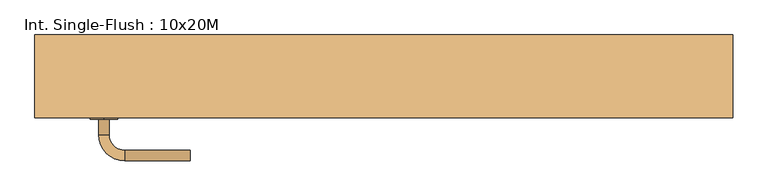
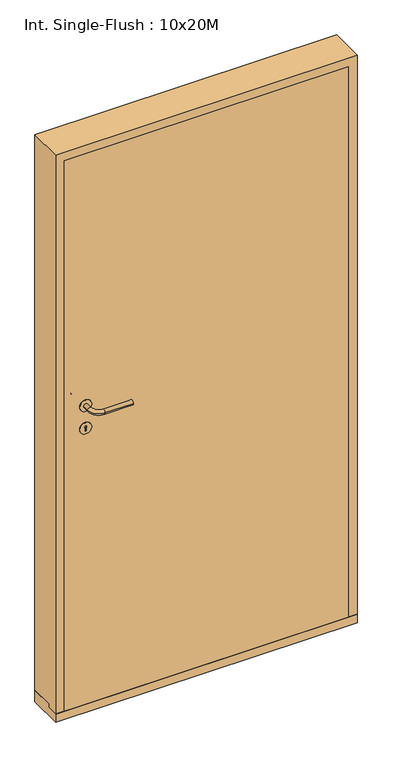
"""IFC4 building model written with IfcOpenShell, lengths in millimetres: door geometry, Int. Single-Flush : 10x20M."""

from ifc_helpers import new_model, si_unit, point, frame, frame_2d, origin, place, context, project, spatial, polyline, circle_curve, ellipse_curve, trimmed, segment, composite_curve, outline, extrude, faceted_brep, source, transform, mapped, element, save
from ifc_brep_helpers import plane_surface, cylinder_surface, revolved_surface, advanced_brep


def int_single_flush_10x20m_68751a9d(model_context):
    return source(origin(), model_context, "Body", "SolidModel", [
        extrude(outline(composite_curve([segment(trimmed(circle_curve(frame_2d((1090.0, -406.0)), 20.0), [point((1070.0, -406.0))], [point((1110.0, -406.0))], False, "CARTESIAN"), True, "CONTINUOUS"), segment(trimmed(circle_curve(frame_2d((1090.0, -406.0)), 20.0), [point((1110.0, -406.0))], [point((1070.0, -406.0))], False, "CARTESIAN"), True, "CONTINUOUS")], self_intersect=False)), frame((0.0, -62.0, 0.0), z_axis=(0.0, 1.0, 0.0), x_axis=(0.0, 0.0, 1.0)), (0.0, 0.0, 1.0), 2.0),
        advanced_brep(
        [(-413.5, -62.0, 1090.0), (-398.5, -62.0, 1090.0), (-398.5, -84.5, 1090.0), (-413.5, -84.5, 1090.0), (-376.0, -107.0, 1090.0), (-376.0, -122.0, 1090.0), (-281.0, -107.0, 1090.0), (-281.0, -122.0, 1090.0)],
        [
            (0, 1, circle_curve(frame((-406.0, -62.0, 1090.0), z_axis=(0.0, 1.0, 0.0), x_axis=(1.0, 0.0, 0.0)), 7.5)),
            (1, 0, circle_curve(frame((-406.0, -62.0, 1090.0), z_axis=(0.0, 1.0, 0.0), x_axis=(1.0, 0.0, 0.0)), 7.5)),
            (1, 2),
            (2, 3, circle_curve(frame((-406.0, -84.5, 1090.0), z_axis=(0.0, 1.0, 0.0), x_axis=(1.0, 0.0, 0.0)), 7.5)),
            (3, 0),
            (3, 2, circle_curve(frame((-406.0, -84.5, 1090.0), z_axis=(0.0, 1.0, 0.0), x_axis=(1.0, 0.0, 0.0)), 7.5)),
            (4, 5, circle_curve(frame((-376.0, -114.5, 1090.0), z_axis=(-1.0, 0.0, 0.0), x_axis=(0.0, 1.0, 0.0)), 7.5)),
            (5, 3, circle_curve(frame((-376.0, -84.5, 1090.0), z_axis=(0.0, 0.0, -1.0), x_axis=(-1.0, 0.0, 0.0)), 37.5)),
            (2, 4, circle_curve(frame((-376.0, -84.5, 1090.0), z_axis=(0.0, 0.0, 1.0), x_axis=(-1.0, 0.0, 0.0)), 22.5)),
            (5, 4, circle_curve(frame((-376.0, -114.5, 1090.0), z_axis=(-1.0, 0.0, 0.0), x_axis=(0.0, 1.0, 0.0)), 7.5)),
            (4, 6),
            (6, 7, circle_curve(frame((-281.0, -114.5, 1090.0), z_axis=(-1.0, 0.0, 0.0), x_axis=(0.0, 1.0, 0.0)), 7.5)),
            (7, 5),
            (7, 6, circle_curve(frame((-281.0, -114.5, 1090.0), z_axis=(-1.0, 0.0, 0.0), x_axis=(0.0, 1.0, 0.0)), 7.5)),
        ],
        [
            plane_surface(frame((-406.0, -62.0, 1090.0), z_axis=(0.0, 1.0, 0.0), x_axis=(0.0, 0.0, -1.0))),
            cylinder_surface(frame((-406.0, -62.0, 1090.0), z_axis=(0.0, 1.0, 0.0), x_axis=(1.0, 0.0, 0.0)), 7.5),
            revolved_surface(trimmed(ellipse_curve(frame((-406.0, -84.5, 1090.0), z_axis=(0.0, -1.0, 0.0), x_axis=(1.0, 0.0, 0.0)), 7.5, 7.5), [point((-413.5, -84.5, 1090.0))], [point((-398.5, -84.5, 1090.0))], True, "CARTESIAN"), (-376.0, -84.5, 1090.0), (0.0, 0.0, -1.0)),
            revolved_surface(trimmed(ellipse_curve(frame((-406.0, -84.5, 1090.0), z_axis=(0.0, -1.0, 0.0), x_axis=(1.0, 0.0, 0.0)), 7.5, 7.5), [point((-398.5, -84.5, 1090.0))], [point((-413.5, -84.5, 1090.0))], True, "CARTESIAN"), (-376.0, -84.5, 1090.0), (0.0, 0.0, -1.0)),
            cylinder_surface(frame((-376.0, -114.5, 1090.0), z_axis=(-1.0, 0.0, 0.0), x_axis=(0.0, 1.0, 0.0)), 7.5),
            plane_surface(frame((-281.0, -114.5, 1090.0), z_axis=(1.0, 0.0, 0.0), x_axis=(0.0, 0.0, -1.0))),
        ],
        [
            (0, [[1, 2]]),
            (1, [[3, 4, 5, -2]]),
            (1, [[-5, 6, -3, -1]]),
            (2, [[7, 8, -4, 9]]),
            (3, [[10, -9, -6, -8]]),
            (4, [[11, 12, 13, -7]]),
            (4, [[-13, 14, -11, -10]]),
            (5, [[-12, -14]]),
        ],
    ),
        extrude(outline(composite_curve([segment(trimmed(circle_curve(frame_2d((1010.0, -406.0)), 20.0), [point((990.0, -406.0))], [point((1030.0, -406.0))], False, "CARTESIAN"), True, "CONTINUOUS"), segment(trimmed(circle_curve(frame_2d((1010.0, -406.0)), 20.0), [point((1030.0, -406.0))], [point((990.0, -406.0))], False, "CARTESIAN"), True, "CONTINUOUS")], self_intersect=False), holes=[composite_curve([segment(trimmed(circle_curve(frame_2d((1015.0, -406.0)), 3.0), [point((1012.4019238, -407.5))], [point((1012.4019238, -404.5))], True, "CARTESIAN"), True, "CONTINUOUS"), segment(polyline([(1012.4019238, -404.5), (1000.0, -404.5), (1000.0, -407.5), (1012.4019238, -407.5)]), True, "CONTINUOUS")], self_intersect=False)]), frame((0.0, -62.0, 0.0), z_axis=(0.0, 1.0, 0.0), x_axis=(0.0, 0.0, 1.0)), (0.0, 0.0, 1.0), 2.0),
        extrude(outline(composite_curve([segment(trimmed(circle_curve(frame_2d((1090.0, -406.0)), 20.0), [point((1070.0, -406.0))], [point((1110.0, -406.0))], False, "CARTESIAN"), True, "CONTINUOUS"), segment(trimmed(circle_curve(frame_2d((1090.0, -406.0)), 20.0), [point((1110.0, -406.0))], [point((1070.0, -406.0))], False, "CARTESIAN"), True, "CONTINUOUS")], self_intersect=False)), frame((0.0, -20.0, 0.0), z_axis=(0.0, 1.0, 0.0), x_axis=(0.0, 0.0, 1.0)), (0.0, 0.0, 1.0), 2.0),
        advanced_brep(
        [(-413.5, -18.0, 1090.0), (-398.5, -18.0, 1090.0), (-413.5, 4.5, 1090.0), (-398.5, 4.5, 1090.0), (-376.0, 27.0, 1090.0), (-376.0, 42.0, 1090.0), (-281.0, 42.0, 1090.0), (-281.0, 27.0, 1090.0)],
        [
            (0, 1, circle_curve(frame((-406.0, -18.0, 1090.0), z_axis=(0.0, -1.0, 0.0), x_axis=(1.0, 0.0, 0.0)), 7.5)),
            (1, 0, circle_curve(frame((-406.0, -18.0, 1090.0), z_axis=(0.0, -1.0, 0.0), x_axis=(1.0, 0.0, 0.0)), 7.5)),
            (0, 2),
            (2, 3, circle_curve(frame((-406.0, 4.5, 1090.0), z_axis=(0.0, -1.0, 0.0), x_axis=(1.0, 0.0, 0.0)), 7.5)),
            (3, 1),
            (3, 2, circle_curve(frame((-406.0, 4.5, 1090.0), z_axis=(0.0, -1.0, 0.0), x_axis=(1.0, 0.0, 0.0)), 7.5)),
            (4, 3, circle_curve(frame((-376.0, 4.5, 1090.0), z_axis=(0.0, 0.0, 1.0), x_axis=(-1.0, 0.0, 0.0)), 22.5)),
            (2, 5, circle_curve(frame((-376.0, 4.5, 1090.0), z_axis=(0.0, 0.0, -1.0), x_axis=(-1.0, 0.0, 0.0)), 37.5)),
            (5, 4, circle_curve(frame((-376.0, 34.5, 1090.0), z_axis=(-1.0, 0.0, 0.0), x_axis=(0.0, -1.0, 0.0)), 7.5)),
            (4, 5, circle_curve(frame((-376.0, 34.5, 1090.0), z_axis=(-1.0, 0.0, 0.0), x_axis=(0.0, -1.0, 0.0)), 7.5)),
            (5, 6),
            (6, 7, circle_curve(frame((-281.0, 34.5, 1090.0), z_axis=(-1.0, 0.0, 0.0), x_axis=(0.0, -1.0, 0.0)), 7.5)),
            (7, 4),
            (7, 6, circle_curve(frame((-281.0, 34.5, 1090.0), z_axis=(-1.0, 0.0, 0.0), x_axis=(0.0, -1.0, 0.0)), 7.5)),
        ],
        [
            plane_surface(frame((-406.0, -18.0, 1090.0), z_axis=(0.0, -1.0, 0.0), x_axis=(0.0, 0.0, -1.0))),
            cylinder_surface(frame((-406.0, -18.0, 1090.0), z_axis=(0.0, -1.0, 0.0), x_axis=(1.0, 0.0, 0.0)), 7.5),
            revolved_surface(trimmed(ellipse_curve(frame((-406.0, 4.5, 1090.0), z_axis=(0.0, -1.0, 0.0), x_axis=(1.0, 0.0, 0.0)), 7.5, 7.5), [point((-413.5, 4.5, 1090.0))], [point((-398.5, 4.5, 1090.0))], True, "CARTESIAN"), (-376.0, 4.5, 1090.0), (0.0, 0.0, -1.0)),
            revolved_surface(trimmed(ellipse_curve(frame((-406.0, 4.5, 1090.0), z_axis=(0.0, -1.0, 0.0), x_axis=(1.0, 0.0, 0.0)), 7.5, 7.5), [point((-398.5, 4.5, 1090.0))], [point((-413.5, 4.5, 1090.0))], True, "CARTESIAN"), (-376.0, 4.5, 1090.0), (0.0, 0.0, -1.0)),
            cylinder_surface(frame((-376.0, 34.5, 1090.0), z_axis=(-1.0, 0.0, 0.0), x_axis=(0.0, -1.0, 0.0)), 7.5),
            plane_surface(frame((-281.0, 34.5, 1090.0), z_axis=(1.0, 0.0, 0.0), x_axis=(0.0, 0.0, -1.0))),
        ],
        [
            (0, [[1, 2]]),
            (1, [[-1, 3, 4, 5]]),
            (1, [[-2, -5, 6, -3]]),
            (2, [[7, -4, 8, 9]]),
            (3, [[-8, -6, -7, 10]]),
            (4, [[-9, 11, 12, 13]]),
            (4, [[-10, -13, 14, -11]]),
            (5, [[-14, -12]]),
        ],
    ),
        extrude(outline(composite_curve([segment(trimmed(circle_curve(frame_2d((1010.0, -406.0)), 20.0), [point((990.0, -406.0))], [point((1030.0, -406.0))], False, "CARTESIAN"), True, "CONTINUOUS"), segment(trimmed(circle_curve(frame_2d((1010.0, -406.0)), 20.0), [point((1030.0, -406.0))], [point((990.0, -406.0))], False, "CARTESIAN"), True, "CONTINUOUS")], self_intersect=False), holes=[composite_curve([segment(trimmed(circle_curve(frame_2d((1015.0, -406.0)), 3.0), [point((1012.4019238, -407.5))], [point((1012.4019238, -404.5))], True, "CARTESIAN"), True, "CONTINUOUS"), segment(polyline([(1012.4019238, -404.5), (1000.0, -404.5), (1000.0, -407.5), (1012.4019238, -407.5)]), True, "CONTINUOUS")], self_intersect=False)]), frame((0.0, -20.0, 0.0), z_axis=(0.0, 1.0, 0.0), x_axis=(0.0, 0.0, 1.0)), (0.0, 0.0, 1.0), 2.0),
        extrude(outline(polyline([(476.0, -20.0), (476.0, -60.0), (-476.0, -60.0), (-476.0, -20.0), (476.0, -20.0)])), frame((0.0, 0.0, 30.0), z_axis=(0.0, 0.0, 1.0), x_axis=(1.0, 0.0, 0.0)), (0.0, 0.0, 1.0), 1952.0),
        extrude(outline(polyline([(-20.0, 42.0), (60.0, 42.0), (60.0, 0.0), (-60.0, 0.0), (-60.0, 30.0), (-20.0, 30.0), (-20.0, 42.0)])), frame((-506.0, 0.0, 0.0), z_axis=(1.0, 0.0, 0.0), x_axis=(0.0, 1.0, 0.0)), (0.0, 0.0, 1.0), 1012.0),
        faceted_brep([(-476.0, -20.0, 1982.0), (-476.0, -20.0, 42.0), (-464.0, -20.0, 42.0), (-464.0, -20.0, 1970.0), (464.0, -20.0, 1970.0), (464.0, -20.0, 42.0), (476.0, -20.0, 42.0), (476.0, -20.0, 1982.0), (-476.0, -60.0, 1982.0), (-476.0, -60.0, 30.0), (-476.0, -20.0, 30.0), (-506.0, -20.0, 30.0), (-506.0, -20.0, 42.0), (506.0, -20.0, 42.0), (506.0, -20.0, 30.0), (476.0, -20.0, 30.0), (-506.0, -60.0, 30.0), (506.0, -60.0, 30.0), (476.0, -60.0, 30.0), (-506.0, -60.0, 2012.0), (476.0, -60.0, 1982.0), (506.0, -60.0, 2012.0), (464.0, 60.0, 42.0), (506.0, 60.0, 42.0), (-506.0, 60.0, 42.0), (-464.0, 60.0, 42.0), (464.0, 60.0, 1970.0), (-464.0, 60.0, 1970.0), (-506.0, 60.0, 2012.0), (506.0, 60.0, 2012.0)], [[[0, 1, 2, 3, 4, 5, 6, 7]], [[8, 9, 10, 1, 0]], [[1, 10, 11, 12]], [[13, 14, 15, 6]], [[10, 9, 16, 11]], [[14, 17, 18, 15]], [[19, 16, 9, 8, 20, 18, 17, 21]], [[7, 6, 15, 18, 20]], [[6, 5, 22, 23, 13]], [[12, 24, 25, 2, 1]], [[26, 22, 5, 4]], [[3, 2, 25, 27]], [[27, 25, 24, 28, 29, 23, 22, 26]], [[21, 17, 14, 13, 23, 29]], [[28, 24, 12, 11, 16, 19]], [[0, 7, 20, 8]], [[3, 27, 26, 4]], [[28, 19, 21, 29]]]),
    ])


if __name__ == "__main__":
    model = new_model("IFC4")
    model_context = context("Model", 3, world=origin())
    ifc_project = project(units=[si_unit("LENGTHUNIT", "METRE", prefix="MILLI")], contexts=[model_context])
    site = spatial("IfcSite", under=ifc_project)
    building = spatial("IfcBuilding", under=site)
    placement = place(None, origin())
    int_single_flush_10x20m_shape = int_single_flush_10x20m_68751a9d(model_context)
    element("IfcDoor", 1, ObjectType="Int. Single-Flush : 10x20M", at=placement, inside=building, context=model_context, shape_type="MappedRepresentation", body=[
        mapped(int_single_flush_10x20m_shape, transform((0.0, 0.0, 0.0), x_axis=(1.0, 0.0, 0.0), y_axis=(0.0, 1.0, 0.0), z_axis=(0.0, 0.0, 1.0))),
    ])
    save(model, "model.ifc")

# Revit data of these elements
# Type "Int. Single-Flush : 10x20M"
#   Type Mark = "73"
#   Sound Rating = ""
#   Hinge Side [instance default] = ""
#   Creator Organization [instance default] = "© Danish Educational Content"
#   Creator Name [instance default] = "© Erik Falck Jørgensen"
#   Creator Build [instance default] = "2017.0801.0"
#   Analytic Construction = "<None>"
#   length#5 = 1012 mm
#   length#3 = 42 mm
#   length#2b = 12 mm
#   length#2a = 0 mm
#   length#2 = 0 mm
#   length#1a = 12 mm
#   length#1 = 0 mm
#   length#4 = 30 mm
#   Thickness = 40 mm
#   Seal Width = 12 mm
#   Rough Width = 1012 mm
#   Rough Height = 2012 mm
#   Rabbet Depth = 40 mm
#   Interior Distance [instance default] = 0 mm
#   Height = 1988 mm
#   Width = 988 mm
#   Handle From Side = 100 mm
#   Handle From Bottom = 1090 mm
#   Exterior Direction [instance default] = 0.00°
#   Case Depth [instance default] = 200 mm
#   Case Width = 30 mm
#   Rabbet Width = 12 mm
#   Exterior Distance [instance default] = 0 mm
#   Bottom Seal = 12 mm
#   Threshold = yes
#   Sealing = no
#   Hinging = yes
#   Wall Closure = 1
#   Door Panel = no
#   Panel = none
#   Handle Finish = none
#   Handle = element 510752
#   Case/Transom = none
#   Function = (empty or 0)
#   Assembly Code = ""
# Element 1 (IfcDoor, "Int. Single-Flush : 10x20M")
#   Case Depth = 120 mm
#   Materials on its faces: "Stainless Steel, Polished", "Default Frame/Mullion (Interior/Exterior)", "Default Door Panel (Exterior/Interior)"
# Materials
#   "Stainless Steel, Polished": class "Metal", colour RGB 180 180 180, transparency 0, Description = "Rustfri stål, poleret", Cost = 0
#   "Default Frame/Mullion (Interior/Exterior)": class "Generic", colour RGB 205 205 205, transparency 0, Description = "Udefineret karm/ramme materiale", Cost = 0
#   "Default Door Panel (Exterior/Interior)": class "Generic", colour RGB 205 205 205, transparency 0, Description = "Udefineret dørplade materiale", Cost = 0
